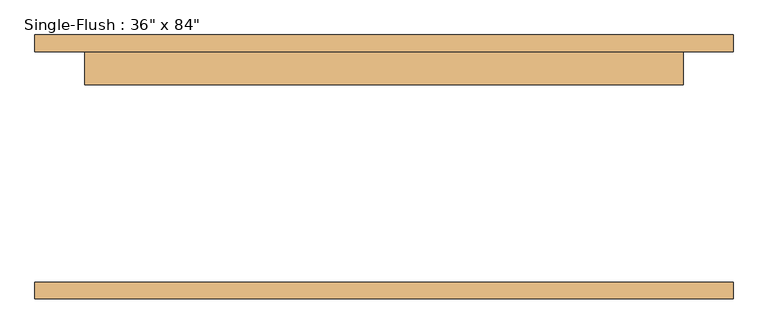
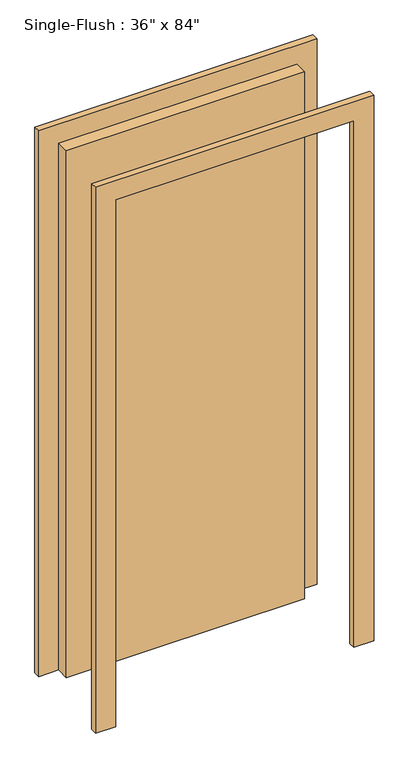
"""IFC4 building model written with IfcOpenShell, lengths in millimetres: door geometry."""

from ifc_helpers import new_model, si_unit, frame, origin, origin_with_axes, place, context, project, spatial, polyline, outline, extrude, source, transform, mapped, element, save


def door_632be17d(model_context):
    return source(origin(), model_context, "Body", "SweptSolid", [
        extrude(outline(polyline([(2209.8, -533.4), (0.0, -533.4), (0.0, -457.2), (2133.6, -457.2), (2133.6, 457.2), (0.0, 457.2), (0.0, 533.4), (2209.8, 533.4), (2209.8, -533.4)])), frame((0.0, 176.2125, 0.0), z_axis=(0.0, 1.0, 0.0), x_axis=(0.0, 0.0, 1.0)), (0.0, 0.0, 1.0), 25.4),
        extrude(outline(polyline([(2209.8, 533.4), (2209.8, -533.4), (0.0, -533.4), (0.0, -457.2), (2133.6, -457.2), (2133.6, 457.2), (0.0, 457.2), (0.0, 533.4), (2209.8, 533.4)])), frame((0.0, -201.6125, 0.0), z_axis=(0.0, 1.0, 0.0), x_axis=(0.0, 0.0, 1.0)), (0.0, 0.0, 1.0), 25.4),
        extrude(outline(polyline([(457.2, 125.4125), (-457.2, 125.4125), (-457.2, 176.2125), (457.2, 176.2125), (457.2, 125.4125)])), origin_with_axes(), (0.0, 0.0, 1.0), 2133.6),
    ])


if __name__ == "__main__":
    model = new_model("IFC4")
    model_context = context("Model", 3, world=origin())
    ifc_project = project(units=[si_unit("LENGTHUNIT", "METRE", prefix="MILLI")], contexts=[model_context])
    site = spatial("IfcSite", under=ifc_project)
    building = spatial("IfcBuilding", under=site)
    placement = place(None, origin())
    door_shape = door_632be17d(model_context)
    element("IfcDoor", 1, ObjectType="Single-Flush : 36\" x 84\"", at=placement, inside=building, context=model_context, shape_type="MappedRepresentation", body=[
        mapped(door_shape, transform((0.0, 0.0, 0.0), x_axis=(1.0, 0.0, 0.0), y_axis=(0.0, 1.0, 0.0), z_axis=(0.0, 0.0, 1.0))),
    ])
    save(model, "model.ifc")

# Revit data of these elements
# Type "Single-Flush : 36\" x 84\""
#   Type Mark = "9"
#   Fire Rating = "--"
#   Assembly Code = "C1020"
#   Thickness = 50.8 mm
#   Height = 2133.6 mm
#   Trim Projection Ext = 25.4 mm
#   Trim Projection Int = 25.4 mm
#   Trim Width = 76.2 mm
#   Width = 914.4 mm
#   Define Thermal Properties by = 0
#   Door Material = Door - Panel
#   Frame Material = Door - Frame
#   Function = (empty or 0)
#   Wall Closure = (empty or 0)
# Element 1 (IfcDoor, "Single-Flush : 36\" x 84\"")
#   Materials on its faces: "Door - Frame", "Door - Panel"
# Materials
#   "Door - Panel": class "Wood", colour RGB 210 159 95, transparency 0, Cost = 0
#   "Door - Frame": class "Miscellaneous", colour RGB 118 70 51, transparency 0, Cost = 0
